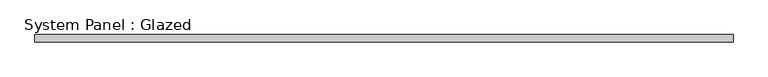
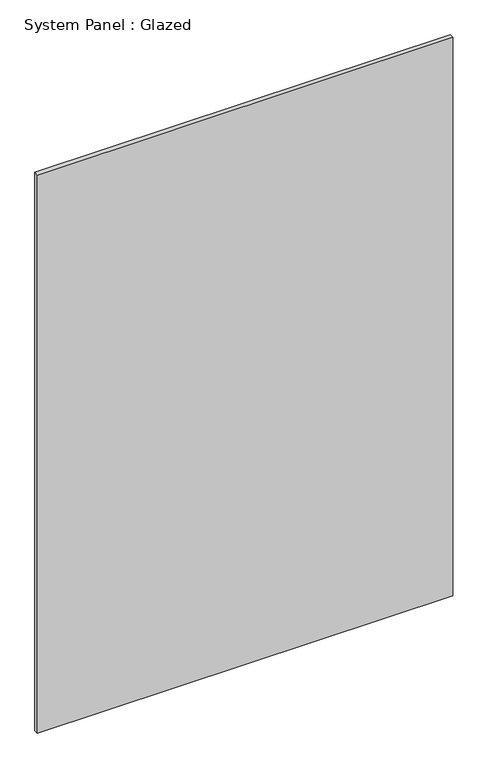
"""IFC4 building model written with IfcOpenShell, lengths in millimetres: plate geometry, System Panel : Glazed."""

from ifc_helpers import new_model, si_unit, origin, origin_with_axes, place, context, project, spatial, polyline, outline, extrude, source, transform, mapped, element, save


def system_panel_glazed_e4114e99(model_context):
    return source(origin(), model_context, "Body", "SweptSolid", [
        extrude(outline(polyline([(1186.5341591, 24.5), (-1186.5341591, 24.5), (-1186.5341591, 49.5), (1186.5341591, 49.5), (1186.5341591, 24.5)])), origin_with_axes(), (0.0, 0.0, 1.0), 3370.0),
    ])


if __name__ == "__main__":
    model = new_model("IFC4")
    model_context = context("Model", 3, world=origin())
    ifc_project = project(units=[si_unit("LENGTHUNIT", "METRE", prefix="MILLI")], contexts=[model_context])
    site = spatial("IfcSite", under=ifc_project)
    building = spatial("IfcBuilding", under=site)
    placement = place(None, origin())
    system_panel_glazed_shape = system_panel_glazed_e4114e99(model_context)
    element("IfcPlate", 1, ObjectType="System Panel : Glazed", at=placement, inside=building, context=model_context, shape_type="MappedRepresentation", body=[
        mapped(system_panel_glazed_shape, transform((0.0, 0.0, 0.0), x_axis=(1.0, 0.0, 0.0), y_axis=(0.0, 1.0, 0.0), z_axis=(0.0, 0.0, 1.0))),
    ])
    save(model, "model.ifc")

# Revit data of these elements
# Type "System Panel : Glazed"
#   Construction Type Id = "GSP4R"
#   Analytic Construction = "1/8 in Pilkington single glazing"
#   Visual Light Transmittance = 0.9
#   Solar Heat Gain Coefficient = 0.86
#   Heat Transfer Coefficient (U) = 6.7069 W/(m²·K)
#   Define Thermal Properties by = 1
# Element 1 (IfcPlate, "System Panel : Glazed")
#   Materials on its faces: "Glass"
# Materials
#   "Glass": class "Glass", colour RGB 245 245 243, transparency 1, Description = "Soda Lime Glass", Cost = 0
